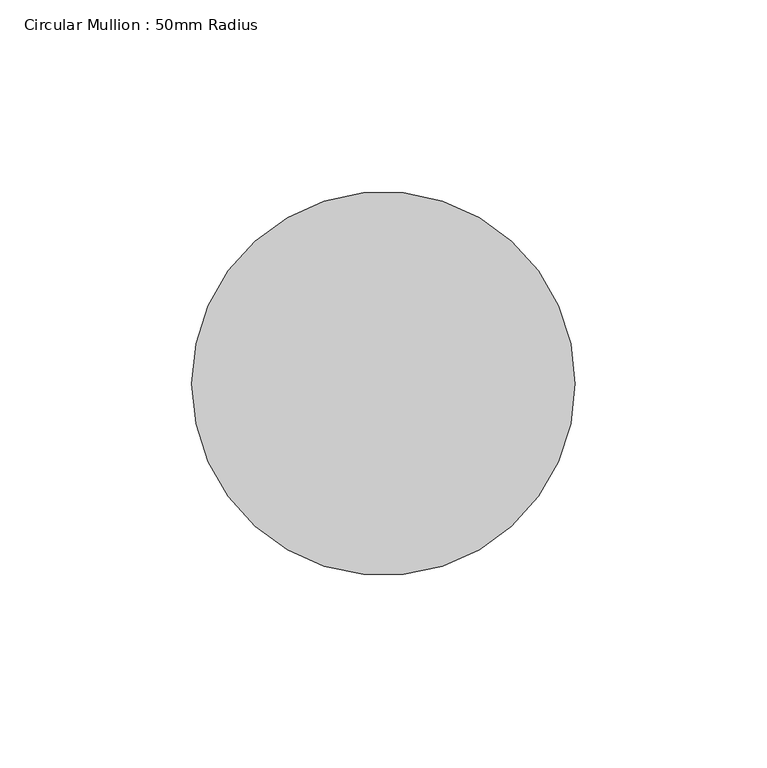
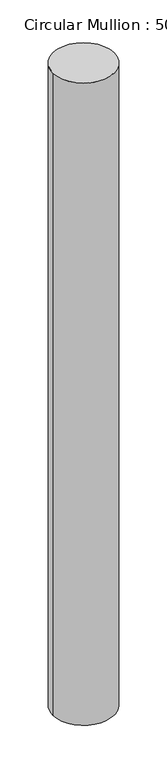
"""IFC4 building model written with IfcOpenShell, lengths in millimetres: member geometry, Circular Mullion : 50mm Radius."""

from ifc_helpers import new_model, si_unit, point, frame, origin, origin_2d, place, context, project, spatial, circle_curve, trimmed, segment, composite_curve, outline, extrude, source, transform, mapped, element, save


def circular_mullion_50mm_radius_09855242(model_context):
    return source(origin(), model_context, "Body", "SweptSolid", [
        extrude(outline(composite_curve([segment(trimmed(circle_curve(origin_2d(), 50.0), [point((50.0, 0.0))], [point((-50.0, 0.0))], False, "CARTESIAN"), True, "CONTINUOUS"), segment(trimmed(circle_curve(origin_2d(), 50.0), [point((-50.0, 0.0))], [point((50.0, 0.0))], False, "CARTESIAN"), True, "CONTINUOUS")], self_intersect=False)), frame((0.0, 0.0, -1111.037899), z_axis=(0.0, 0.0, 1.0), x_axis=(1.0, 0.0, 0.0)), (0.0, 0.0, 1.0), 1111.037899),
    ])


if __name__ == "__main__":
    model = new_model("IFC4")
    model_context = context("Model", 3, world=origin())
    ifc_project = project(units=[si_unit("LENGTHUNIT", "METRE", prefix="MILLI")], contexts=[model_context])
    site = spatial("IfcSite", under=ifc_project)
    building = spatial("IfcBuilding", under=site)
    placement = place(None, origin())
    circular_mullion_50mm_radius_shape = circular_mullion_50mm_radius_09855242(model_context)
    element("IfcMember", 1, ObjectType="Circular Mullion : 50mm Radius", at=placement, inside=building, context=model_context, shape_type="MappedRepresentation", body=[
        mapped(circular_mullion_50mm_radius_shape, transform((0.0, 0.0, 0.0), x_axis=(1.0, 0.0, 0.0), y_axis=(0.0, 1.0, 0.0), z_axis=(0.0, 0.0, 1.0))),
    ])
    save(model, "model.ifc")

# Revit data of these elements
# Type "Circular Mullion : 50mm Radius"
#   built-in parameter 1007350 = 0.164042 (stored number, unit not read)
# Element 1 (IfcMember, "Circular Mullion : 50mm Radius")
#   Materials on its faces: "Aluminium"
# Materials
#   "Aluminium": class "Metal", colour RGB 247 247 247, transparency 0, Description = "Aluminium 6061", Cost = 0
